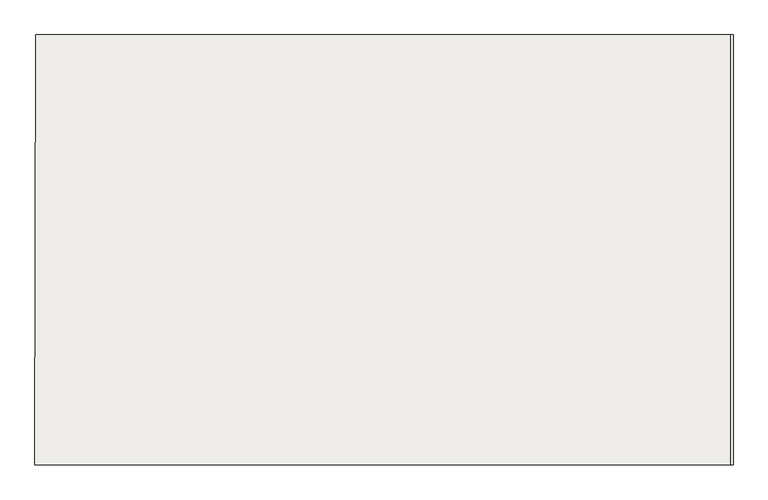
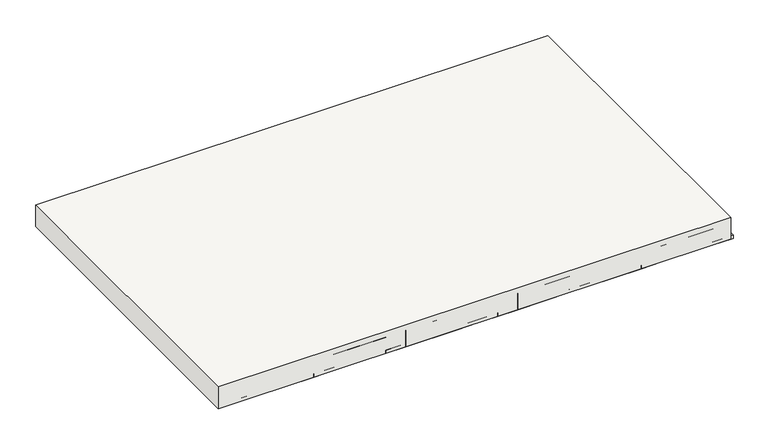
"""IFC4 building model written with IfcOpenShell, lengths in millimetres: slab geometry, Pano 1 (16 cm)."""

import ifcopenshell
import ifcopenshell.guid

model = None  # the IFC model being written
_history = None  # IfcOwnerHistory: only IFC2X3 demands one
_inside = {}  # id of a spatial element -> (the spatial element, [elements in it])
_under = {}  # id of a project, library or spatial element -> (it, [spatial elements below it])
_declared = {}  # id of a project -> (the project, [libraries it declares])
_typed = {}  # id of a type object -> (the type object, [elements of that type])
_made_of = {}  # id of a material, layer set ... -> (it, [elements and type objects made of it])


def new_model(schema):
    """Start an empty IFC model of exactly this schema.

    Asked for "IFC4X3", IfcOpenShell would pick the latest addendum, in which some entities
    have other attributes; the version numbers below select the first issue.
    IFC2X3 requires an IfcOwnerHistory on every rooted entity: one is made here for all.
    """
    global model, _history
    if schema == "IFC4X3":
        model = ifcopenshell.file(schema_version=(4, 3, 0, 0))
    else:
        model = ifcopenshell.file(schema=schema)
    _inside.clear()
    _under.clear()
    _declared.clear()
    _typed.clear()
    _made_of.clear()
    _history = None
    if model.schema == "IFC2X3":
        org = make("IfcOrganization", Name="unknown")
        user = make(
            "IfcPersonAndOrganization",
            ThePerson=make("IfcPerson", FamilyName="unknown"),
            TheOrganization=org,
        )
        app = make(
            "IfcApplication",
            ApplicationDeveloper=org,
            Version="unknown",
            ApplicationFullName="unknown",
            ApplicationIdentifier="unknown",
        )
        _history = make(
            "IfcOwnerHistory",
            OwningUser=user,
            OwningApplication=app,
            ChangeAction="ADDED",
            CreationDate=0,
        )
    return model


def make(cls, **values):
    """One entity of the class cls with the attributes given. An attribute that is None is left unset."""
    return model.create_entity(
        cls, **{name: value for name, value in values.items() if value is not None}
    )


def rooted(cls, **values):
    """An entity with a GlobalId (a new one), such as an element, a storey or a relation."""
    return make(cls, GlobalId=ifcopenshell.guid.new(), OwnerHistory=_history, **values)


def si_unit(unit_type, name, prefix=None):
    """IfcSIUnit, for example si_unit("LENGTHUNIT", "METRE", prefix="MILLI")."""
    return make("IfcSIUnit", UnitType=unit_type, Prefix=prefix, Name=name)


def assignment(units):
    """IfcUnitAssignment: the units of a project."""
    return None if units is None else make("IfcUnitAssignment", Units=units)


def point(xyz):
    """IfcCartesianPoint."""
    return None if xyz is None else make("IfcCartesianPoint", Coordinates=xyz)


def direction(xyz):
    """IfcDirection."""
    return None if xyz is None else make("IfcDirection", DirectionRatios=xyz)


def frame(location, z_axis=None, x_axis=None):
    """IfcAxis2Placement3D, a coordinate frame: its origin and axes. An axis left out is left unset."""
    return make(
        "IfcAxis2Placement3D",
        Location=point(location),
        Axis=direction(z_axis),
        RefDirection=direction(x_axis),
    )


def origin():
    """The frame at (0, 0, 0) with its axes left unset."""
    return frame((0.0, 0.0, 0.0))


def origin_with_axes():
    """The frame at (0, 0, 0) with the z axis (0, 0, 1) and the x axis (1, 0, 0) written out."""
    return frame((0.0, 0.0, 0.0), z_axis=(0.0, 0.0, 1.0), x_axis=(1.0, 0.0, 0.0))


def place(relative_to, where):
    """IfcLocalPlacement: puts the frame where relative to a parent placement (None: the world)."""
    return make(
        "IfcLocalPlacement", PlacementRelTo=relative_to, RelativePlacement=where
    )


def context(
    kind, dimensions, precision=None, world=None, true_north=None, identifier=None
):
    """IfcGeometricRepresentationContext, for example the 3D "Model" context."""
    return make(
        "IfcGeometricRepresentationContext",
        ContextIdentifier=identifier,
        ContextType=kind,
        CoordinateSpaceDimension=dimensions,
        Precision=precision,
        WorldCoordinateSystem=world,
        TrueNorth=true_north,
    )


def project(units=None, contexts=None):
    """IfcProject with its units and contexts."""
    return rooted(
        "IfcProject",
        Name="project",
        RepresentationContexts=contexts,
        UnitsInContext=assignment(units),
    )


def spatial(cls, under=None, at=None, **own):
    """A site, building, storey or space (cls), placed at a placement, below another one or the project."""
    s = rooted(cls, ObjectPlacement=at, **own)
    if under is not None:
        _under.setdefault(under.id(), (under, []))[1].append(s)
    return s


def polyline(points):
    """IfcPolyline through the points."""
    return make("IfcPolyline", Points=[point(p) for p in points])


def outline(outer, holes=None, kind="AREA"):
    """IfcArbitraryClosedProfileDef: a profile drawn as a closed curve; with holes, ...WithVoids."""
    if holes is None:
        return make("IfcArbitraryClosedProfileDef", ProfileType=kind, OuterCurve=outer)
    return make(
        "IfcArbitraryProfileDefWithVoids",
        ProfileType=kind,
        OuterCurve=outer,
        InnerCurves=holes,
    )


def extrude(swept, where, along, depth):
    """IfcExtrudedAreaSolid: the profile swept, set in the frame where, extruded along a direction by depth."""
    return make(
        "IfcExtrudedAreaSolid",
        SweptArea=swept,
        Position=where,
        ExtrudedDirection=direction(along),
        Depth=depth,
    )


def shape(context_of_items, identifier, shape_type, items):
    """IfcShapeRepresentation: the items that make up one representation, for example the "Body"."""
    return make(
        "IfcShapeRepresentation",
        ContextOfItems=context_of_items,
        RepresentationIdentifier=identifier,
        RepresentationType=shape_type,
        Items=items,
    )


def source(mapping_origin, context_of_items, identifier, shape_type, items):
    """IfcRepresentationMap: a shape defined once, which mapped items show again and again."""
    return make(
        "IfcRepresentationMap",
        MappingOrigin=mapping_origin,
        MappedRepresentation=shape(context_of_items, identifier, shape_type, items),
    )


def transform(
    local_origin,
    x_axis=None,
    y_axis=None,
    z_axis=None,
    scale=None,
    scale2=None,
    scale3=None,
    uniform=True,
):
    """IfcCartesianTransformationOperator3D, or its non-uniform kind. x_axis, y_axis, z_axis: its Axis1, 2, 3."""
    if uniform:
        return make(
            "IfcCartesianTransformationOperator3D",
            Axis1=direction(x_axis),
            Axis2=direction(y_axis),
            LocalOrigin=point(local_origin),
            Scale=scale,
            Axis3=direction(z_axis),
        )
    return make(
        "IfcCartesianTransformationOperator3DnonUniform",
        Axis1=direction(x_axis),
        Axis2=direction(y_axis),
        LocalOrigin=point(local_origin),
        Scale=scale,
        Axis3=direction(z_axis),
        Scale2=scale2,
        Scale3=scale3,
    )


def mapped(mapping_source, mapping_target):
    """IfcMappedItem: shows the shape of a source again, moved by a transform."""
    return make(
        "IfcMappedItem", MappingSource=mapping_source, MappingTarget=mapping_target
    )


def made_of(thing, what):
    """Note that an element or type object is made of a material, layer set ...; save() writes the relation."""
    if what is not None:
        _made_of.setdefault(what.id(), (what, []))[1].append(thing)
    return thing


def element(
    cls,
    number,
    at=None,
    inside=None,
    cuts=None,
    type_object=None,
    material=None,
    context=None,
    identifier="Body",
    shape_type=None,
    held_by="IfcProductDefinitionShape",
    body=None,
    shapes=None,
    **own,
):
    """One element of the class cls, such as IfcWall. Its Tag is "e" and its number.

    at: its placement. inside: the storey or other place that contains it. cuts: it is an
    opening in that element (IfcRelVoidsElement). A single representation is given by context,
    identifier, shape_type and body (its items); several are given by shapes. held_by: the class
    of the entity that holds the representations. save() writes the other relations.
    """
    e = rooted(cls, Tag="e%d" % number, ObjectPlacement=at, **own)
    if body is not None:
        shapes = [shape(context, identifier, shape_type, body)]
    if shapes is not None:
        e.Representation = make(held_by, Representations=shapes)
    if inside is not None:
        _inside.setdefault(inside.id(), (inside, []))[1].append(e)
    if cuts is not None:
        rooted(
            "IfcRelVoidsElement", RelatingBuildingElement=cuts, RelatedOpeningElement=e
        )
    if type_object is not None:
        _typed.setdefault(type_object.id(), (type_object, []))[1].append(e)
    return made_of(e, material)


def aggregate(whole, parts):
    """IfcRelAggregates: a whole, such as a stair, and the parts it consists of."""
    return rooted("IfcRelAggregates", RelatingObject=whole, RelatedObjects=parts)


def save(model, path):
    """Write the relations noted so far, then the file.

    IfcRelAggregates (storeys below a building ...), IfcRelContainedInSpatialStructure (elements
    in a storey), IfcRelDefinesByType, IfcRelAssociatesMaterial and IfcRelDeclares: one each for
    every whole, place, type object, material and project.
    """
    for whole, parts in _under.values():
        aggregate(whole, parts)
    for where, things in _inside.values():
        rooted(
            "IfcRelContainedInSpatialStructure",
            RelatedElements=things,
            RelatingStructure=where,
        )
    for kind, things in _typed.values():
        rooted("IfcRelDefinesByType", RelatedObjects=things, RelatingType=kind)
    for what, things in _made_of.values():
        rooted("IfcRelAssociatesMaterial", RelatedObjects=things, RelatingMaterial=what)
    for by, libraries in _declared.values():
        rooted("IfcRelDeclares", RelatingContext=by, RelatedDefinitions=libraries)
    model.write(path)


def slab_6dcc425b(model_context):
    return source(origin(), model_context, "Body", "SweptSolid", [
        extrude(outline(polyline([(-140.0, 2350.0), (-140.0, 140.0), (-3709.999588, 140.0), (-3704.63551, 2350.0), (-140.0, 2350.0)])), origin_with_axes(), (0.0, 0.0, 1.0), 160.0),
        extrude(outline(polyline([(-3045.0, 1640.0), (-3405.0, 1640.0), (-3405.0, 2135.0), (-3045.0, 2135.0), (-3045.0, 1640.0)])), origin_with_axes(), (0.0, 0.0, 1.0), 120.0),
        extrude(outline(polyline([(-2405.0, 140.0), (-2545.0, 140.0), (-2545.0, 2350.0), (-2405.0, 2350.0), (-2405.0, 140.0)])), origin_with_axes(), (0.0, 0.0, 1.0), 24.0),
        extrude(outline(polyline([(-765.0, 1140.0), (-1125.0, 1140.0), (-1125.0, 1635.0), (-765.0, 1635.0), (-765.0, 1140.0)])), origin_with_axes(), (0.0, 0.0, 1.0), 120.0),
        extrude(outline(polyline([(-2045.0, 2140.0), (-2405.0, 2140.0), (-2405.0, 2345.0), (-2045.0, 2345.0), (-2045.0, 2140.0)])), origin_with_axes(), (0.0, 0.0, 1.0), 120.0),
        extrude(outline(polyline([(-2045.0, 140.0), (-2405.0, 140.0), (-2405.0, 635.0), (-2045.0, 635.0), (-2045.0, 140.0)])), origin_with_axes(), (0.0, 0.0, 1.0), 120.0),
        extrude(outline(polyline([(-2045.0, 1140.0), (-2405.0, 1140.0), (-2405.0, 1635.0), (-2045.0, 1635.0), (-2045.0, 1140.0)])), origin_with_axes(), (0.0, 0.0, 1.0), 120.0),
        extrude(outline(polyline([(-2545.0, 1140.0), (-2905.0, 1140.0), (-2905.0, 1635.0), (-2545.0, 1635.0), (-2545.0, 1140.0)])), origin_with_axes(), (0.0, 0.0, 1.0), 120.0),
        extrude(outline(polyline([(-265.0, 640.0), (-625.0, 640.0), (-625.0, 1135.0), (-265.0, 1135.0), (-265.0, 640.0)])), origin_with_axes(), (0.0, 0.0, 1.0), 120.0),
        extrude(outline(polyline([(-3045.0, 140.0), (-3405.0, 140.0), (-3405.0, 635.0), (-3045.0, 635.0), (-3045.0, 140.0)])), origin_with_axes(), (0.0, 0.0, 1.0), 120.0),
        extrude(outline(polyline([(-2045.0, 640.0), (-2405.0, 640.0), (-2405.0, 1135.0), (-2045.0, 1135.0), (-2045.0, 640.0)])), origin_with_axes(), (0.0, 0.0, 1.0), 120.0),
        extrude(outline(polyline([(-1265.0, 140.0), (-1625.0, 140.0), (-1625.0, 635.0), (-1265.0, 635.0), (-1265.0, 140.0)])), origin_with_axes(), (0.0, 0.0, 1.0), 120.0),
        extrude(outline(polyline([(-765.0, 140.0), (-1125.0, 140.0), (-1125.0, 635.0), (-765.0, 635.0), (-765.0, 140.0)])), origin_with_axes(), (0.0, 0.0, 1.0), 120.0),
        extrude(outline(polyline([(-3045.0, 640.0), (-3405.0, 640.0), (-3405.0, 1135.0), (-3045.0, 1135.0), (-3045.0, 640.0)])), origin_with_axes(), (0.0, 0.0, 1.0), 120.0),
        extrude(outline(polyline([(-765.0, 640.0), (-1125.0, 640.0), (-1125.0, 1135.0), (-765.0, 1135.0), (-765.0, 640.0)])), origin_with_axes(), (0.0, 0.0, 1.0), 120.0),
        extrude(outline(polyline([(-125.0, 140.0), (-265.0, 140.0), (-265.0, 2350.0), (-125.0, 2350.0), (-125.0, 140.0)])), origin_with_axes(), (0.0, 0.0, 1.0), 24.0),
        extrude(outline(polyline([(-765.0, 2140.0), (-1125.0, 2140.0), (-1125.0, 2345.0), (-765.0, 2345.0), (-765.0, 2140.0)])), origin_with_axes(), (0.0, 0.0, 1.0), 120.0),
        extrude(outline(polyline([(-625.0, 140.0), (-765.0, 140.0), (-765.0, 2350.0), (-625.0, 2350.0), (-625.0, 140.0)])), origin_with_axes(), (0.0, 0.0, 1.0), 24.0),
        extrude(outline(polyline([(-1905.0, 140.0), (-2045.0, 140.0), (-2045.0, 2350.0), (-1905.0, 2350.0), (-1905.0, 140.0)])), origin_with_axes(), (0.0, 0.0, 1.0), 24.0),
        extrude(outline(polyline([(-3405.0, 140.0), (-3545.0, 140.0), (-3545.0, 2350.0), (-3405.0, 2350.0), (-3405.0, 140.0)])), origin_with_axes(), (0.0, 0.0, 1.0), 24.0),
        extrude(outline(polyline([(-265.0, 1640.0), (-625.0, 1640.0), (-625.0, 2135.0), (-265.0, 2135.0), (-265.0, 1640.0)])), origin_with_axes(), (0.0, 0.0, 1.0), 120.0),
        extrude(outline(polyline([(-2045.0, 1640.0), (-2405.0, 1640.0), (-2405.0, 2135.0), (-2045.0, 2135.0), (-2045.0, 1640.0)])), origin_with_axes(), (0.0, 0.0, 1.0), 120.0),
        extrude(outline(polyline([(-3045.0, 2140.0), (-3405.0, 2140.0), (-3405.0, 2345.0), (-3045.0, 2345.0), (-3045.0, 2140.0)])), origin_with_axes(), (0.0, 0.0, 1.0), 120.0),
        extrude(outline(polyline([(-265.0, 1140.0), (-625.0, 1140.0), (-625.0, 1635.0), (-265.0, 1635.0), (-265.0, 1140.0)])), origin_with_axes(), (0.0, 0.0, 1.0), 120.0),
        extrude(outline(polyline([(-1765.0, 140.0), (-1905.0, 140.0), (-1905.0, 2350.0), (-1765.0, 2350.0), (-1765.0, 140.0)])), origin_with_axes(), (0.0, 0.0, 1.0), 24.0),
        extrude(outline(polyline([(-2905.0, 140.0), (-3045.0, 140.0), (-3045.0, 2350.0), (-2905.0, 2350.0), (-2905.0, 140.0)])), origin_with_axes(), (0.0, 0.0, 1.0), 24.0),
        extrude(outline(polyline([(-2545.0, 640.0), (-2905.0, 640.0), (-2905.0, 1135.0), (-2545.0, 1135.0), (-2545.0, 640.0)])), origin_with_axes(), (0.0, 0.0, 1.0), 120.0),
        extrude(outline(polyline([(-2545.0, 1640.0), (-2905.0, 1640.0), (-2905.0, 2135.0), (-2545.0, 2135.0), (-2545.0, 1640.0)])), origin_with_axes(), (0.0, 0.0, 1.0), 120.0),
        extrude(outline(polyline([(-1265.0, 640.0), (-1625.0, 640.0), (-1625.0, 1135.0), (-1265.0, 1135.0), (-1265.0, 640.0)])), origin_with_axes(), (0.0, 0.0, 1.0), 120.0),
        extrude(outline(polyline([(-1265.0, 2140.0), (-1625.0, 2140.0), (-1625.0, 2345.0), (-1265.0, 2345.0), (-1265.0, 2140.0)])), origin_with_axes(), (0.0, 0.0, 1.0), 120.0),
        extrude(outline(polyline([(-3045.0, 1140.0), (-3405.0, 1140.0), (-3405.0, 1635.0), (-3045.0, 1635.0), (-3045.0, 1140.0)])), origin_with_axes(), (0.0, 0.0, 1.0), 120.0),
        extrude(outline(polyline([(-765.0, 1640.0), (-1125.0, 1640.0), (-1125.0, 2135.0), (-765.0, 2135.0), (-765.0, 1640.0)])), origin_with_axes(), (0.0, 0.0, 1.0), 120.0),
        extrude(outline(polyline([(-265.0, 2140.0), (-625.0, 2140.0), (-625.0, 2345.0), (-265.0, 2345.0), (-265.0, 2140.0)])), origin_with_axes(), (0.0, 0.0, 1.0), 120.0),
        extrude(outline(polyline([(-2545.0, 2140.0), (-2905.0, 2140.0), (-2905.0, 2345.0), (-2545.0, 2345.0), (-2545.0, 2140.0)])), origin_with_axes(), (0.0, 0.0, 1.0), 120.0),
        extrude(outline(polyline([(-1125.0, 140.0), (-1265.0, 140.0), (-1265.0, 2350.0), (-1125.0, 2350.0), (-1125.0, 140.0)])), origin_with_axes(), (0.0, 0.0, 1.0), 24.0),
        extrude(outline(polyline([(-1265.0, 1640.0), (-1625.0, 1640.0), (-1625.0, 2135.0), (-1265.0, 2135.0), (-1265.0, 1640.0)])), origin_with_axes(), (0.0, 0.0, 1.0), 120.0),
        extrude(outline(polyline([(-1625.0, 140.0), (-1765.0, 140.0), (-1765.0, 2350.0), (-1625.0, 2350.0), (-1625.0, 140.0)])), origin_with_axes(), (0.0, 0.0, 1.0), 24.0),
        extrude(outline(polyline([(-265.0, 140.0), (-625.0, 140.0), (-625.0, 635.0), (-265.0, 635.0), (-265.0, 140.0)])), origin_with_axes(), (0.0, 0.0, 1.0), 120.0),
        extrude(outline(polyline([(-1265.0, 1140.0), (-1625.0, 1140.0), (-1625.0, 1635.0), (-1265.0, 1635.0), (-1265.0, 1140.0)])), origin_with_axes(), (0.0, 0.0, 1.0), 120.0),
        extrude(outline(polyline([(-2545.0, 140.0), (-2905.0, 140.0), (-2905.0, 635.0), (-2545.0, 635.0), (-2545.0, 140.0)])), origin_with_axes(), (0.0, 0.0, 1.0), 120.0),
    ])


if __name__ == "__main__":
    model = new_model("IFC4")
    model_context = context("Model", 3, world=origin())
    ifc_project = project(units=[si_unit("LENGTHUNIT", "METRE", prefix="MILLI")], contexts=[model_context])
    site = spatial("IfcSite", under=ifc_project)
    building = spatial("IfcBuilding", under=site)
    placement = place(None, origin())
    slab_shape = slab_6dcc425b(model_context)
    element("IfcSlab", 1, ObjectType="Pano 1 (16 cm)", at=placement, inside=building, context=model_context, shape_type="MappedRepresentation", body=[
        mapped(slab_shape, transform((0.0, 0.0, 0.0), x_axis=(1.0, 0.0, 0.0), y_axis=(0.0, 1.0, 0.0), z_axis=(0.0, 0.0, 1.0))),
    ])
    save(model, "model.ifc")

# Revit data of these elements
# Element 1 (IfcSlab, "Pano 1 (16 cm)")
#   Materials on its faces: "Molde de poliestireno", "Concreto armado", "RGB 168-169-158"
# Materials
#   "Molde de poliestireno": class "Não atribuído", colour RGB 255 255 255, transparency 0
#   "Concreto armado": class "Não atribuído", colour RGB 168 169 158, transparency 0
#   "RGB 168-169-158": class "Não atribuído", colour RGB 168 169 158, transparency 0
